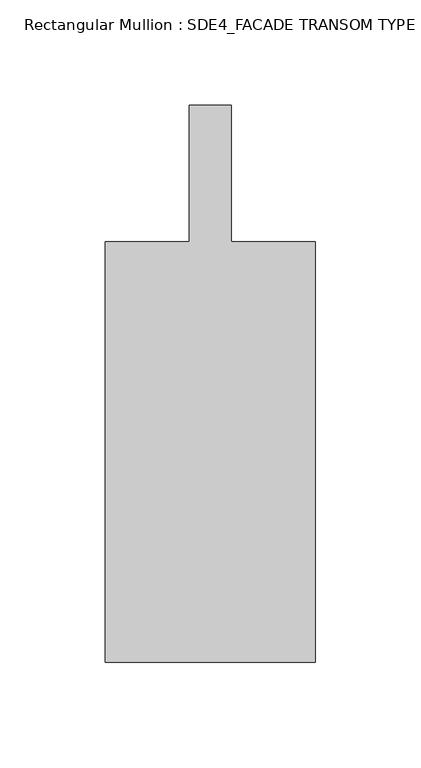
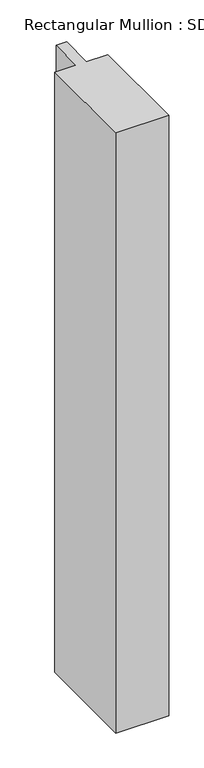
"""IFC4 building model written with IfcOpenShell, lengths in millimetres: member geometry, Rectangular Mullion : SDE4_FACADE TRANSOM TYPE 2."""

from ifc_helpers import new_model, si_unit, frame, origin, place, context, project, spatial, polyline, outline, extrude, source, transform, mapped, element, save


def rectangular_mullion_sde4_facade_transom_type_2_8c3a16e5(model_context):
    return source(origin(), model_context, "Body", "SweptSolid", [
        extrude(outline(polyline([(50.0, -132.5), (-50.0, -132.5), (-50.0, 67.5), (-10.0, 67.5), (-10.0, 132.5), (10.0, 132.5), (10.0, 67.5), (50.0, 67.5), (50.0, -132.5)])), frame((0.0, 0.0, -1200.1002391), z_axis=(0.0, 0.0, 1.0), x_axis=(1.0, 0.0, 0.0)), (0.0, 0.0, 1.0), 1200.1002391),
    ])


if __name__ == "__main__":
    model = new_model("IFC4")
    model_context = context("Model", 3, world=origin())
    ifc_project = project(units=[si_unit("LENGTHUNIT", "METRE", prefix="MILLI")], contexts=[model_context])
    site = spatial("IfcSite", under=ifc_project)
    building = spatial("IfcBuilding", under=site)
    placement = place(None, origin())
    rectangular_mullion_sde4_facade_transom_type_2_shape = rectangular_mullion_sde4_facade_transom_type_2_8c3a16e5(model_context)
    element("IfcMember", 1, ObjectType="Rectangular Mullion : SDE4_FACADE TRANSOM TYPE 2", at=placement, inside=building, context=model_context, shape_type="MappedRepresentation", body=[
        mapped(rectangular_mullion_sde4_facade_transom_type_2_shape, transform((0.0, 0.0, 0.0), x_axis=(1.0, 0.0, 0.0), y_axis=(0.0, 1.0, 0.0), z_axis=(0.0, 0.0, 1.0))),
    ])
    save(model, "model.ifc")

# Revit data of these elements
# Type "Rectangular Mullion : SDE4_FACADE TRANSOM TYPE 2"
#   built-in parameter 1007322 = 0.869423 (stored number, unit not read)
#   built-in parameter 1007321 = 0.164042 (stored number, unit not read)
#   built-in parameter 1007320 = 0.164042 (stored number, unit not read)
